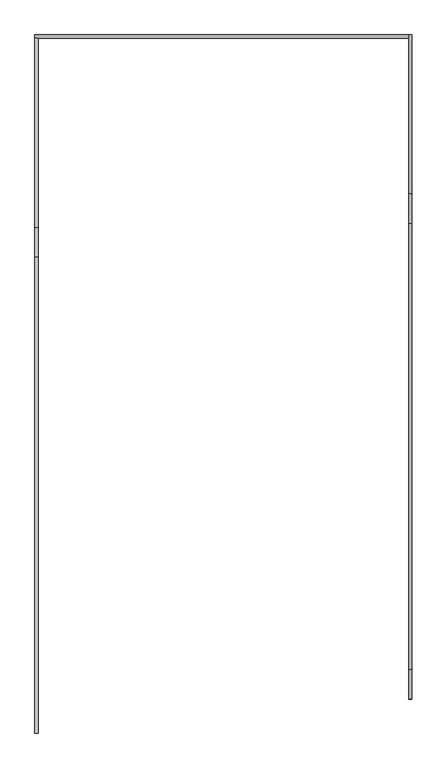
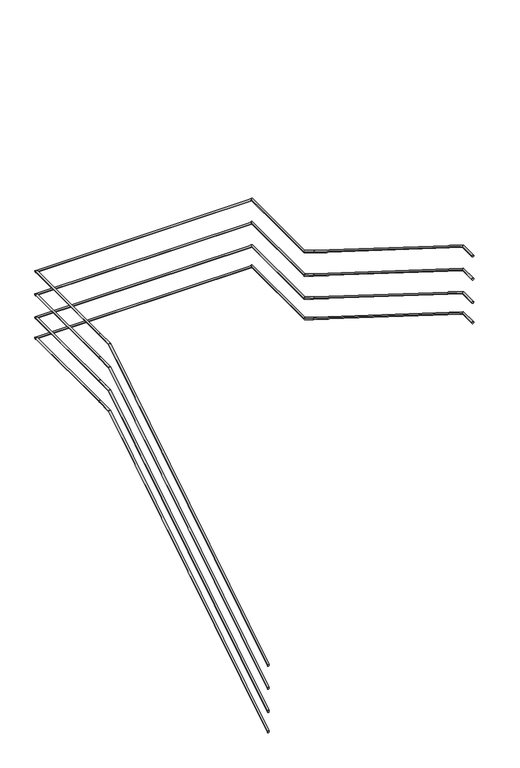
"""IFC4 building model written with IfcOpenShell, lengths in millimetres: railing geometry."""

from ifc_helpers import new_model, si_unit, frame, origin, place, context, project, spatial, circle_curve, ellipse_curve, source, transform, mapped, element, save
from ifc_brep_helpers import plane_surface, cylinder_surface, advanced_brep


def railing_8161422b(model_context):
    return source(origin(), model_context, "Body", "AdvancedBrep", [
        advanced_brep(
        [(51115.4, 10964.5208589, 1508.0091814), (51085.4, 10964.5208589, 1508.0091814), (51115.4, 15448.8385799, 4322.8406512), (51085.4, 15448.8385799, 4322.8406512), (51115.4, 15724.5208589, 4322.8406512), (51085.4, 15724.5208589, 4322.8406512)],
        [
            (0, 1, ellipse_curve(frame((51100.4, 10964.5208589, 1508.0091814), z_axis=(0.0, -1.0, 0.0), x_axis=(0.0, 0.0, -1.0)), 17.7102578, 15.0)),
            (1, 0, ellipse_curve(frame((51100.4, 10964.5208589, 1508.0091814), z_axis=(0.0, -1.0, 0.0), x_axis=(0.0, 0.0, -1.0)), 17.7102578, 15.0)),
            (0, 2),
            (2, 3, ellipse_curve(frame((51100.4, 15448.8385799, 4322.8406512), z_axis=(0.0, -0.9609804318330746, -0.27661635821823227), x_axis=(0.0, 0.27661635821823216, -0.9609804318330747)), 15.6090587, 15.0)),
            (3, 1),
            (3, 2, ellipse_curve(frame((51100.4, 15448.8385799, 4322.8406512), z_axis=(0.0, -0.9609804318330746, -0.27661635821823227), x_axis=(0.0, 0.27661635821823216, -0.9609804318330747)), 15.6090587, 15.0)),
            (4, 5, circle_curve(frame((51100.4, 15724.5208589, 4322.8406512), z_axis=(0.0, 1.0, 0.0), x_axis=(-1.0, 0.0, 0.0)), 15.0)),
            (5, 4, circle_curve(frame((51100.4, 15724.5208589, 4322.8406512), z_axis=(0.0, 1.0, 0.0), x_axis=(-1.0, 0.0, 0.0)), 15.0)),
            (2, 4),
            (5, 3),
        ],
        [
            plane_surface(frame((51100.4, 10964.5208589, 1525.7194391), z_axis=(0.0, -1.0, 0.0), x_axis=(0.0, 0.0, 1.0))),
            cylinder_surface(frame((51100.4, 10972.4955461, 1513.0149374), z_axis=(0.0, -0.8469667807321652, -0.5316458147452987), x_axis=(-1.0, 0.0, 0.0)), 15.0),
            plane_surface(frame((51100.4, 15724.5208589, 4337.8406512), z_axis=(0.0, 1.0, 0.0), x_axis=(0.0, 0.0, 1.0))),
            cylinder_surface(frame((51100.4, 15444.5208589, 4322.8406512), z_axis=(0.0, -1.0, 0.0), x_axis=(-1.0, 0.0, 0.0)), 15.0),
        ],
        [
            (0, [[1, 2]]),
            (1, [[-1, 3, 4, 5]]),
            (1, [[-2, -5, 6, -3]]),
            (2, [[7, 8]]),
            (3, [[-4, 9, -8, 10]]),
            (3, [[-6, -10, -7, -9]]),
        ],
    ),
        advanced_brep(
        [(51115.4, 15724.5208589, 4322.8406512), (51085.4, 15724.5208589, 4322.8406512), (51115.4, 17509.1208589, 4322.8406512), (51085.4, 17509.1208589, 4322.8406512)],
        [
            (0, 1, circle_curve(frame((51100.4, 15724.5208589, 4322.8406512), z_axis=(0.0, -1.0, 0.0), x_axis=(-1.0, 0.0, 0.0)), 15.0)),
            (1, 0, circle_curve(frame((51100.4, 15724.5208589, 4322.8406512), z_axis=(0.0, -1.0, 0.0), x_axis=(-1.0, 0.0, 0.0)), 15.0)),
            (2, 3, circle_curve(frame((51100.4, 17509.1208589, 4322.8406512), z_axis=(0.0, 1.0, 0.0), x_axis=(-1.0, 0.0, 0.0)), 15.0)),
            (3, 2, circle_curve(frame((51100.4, 17509.1208589, 4322.8406512), z_axis=(0.0, 1.0, 0.0), x_axis=(-1.0, 0.0, 0.0)), 15.0)),
            (0, 2),
            (3, 1),
        ],
        [
            plane_surface(frame((51100.4, 15724.5208589, 4337.8406512), z_axis=(0.0, -1.0, 0.0), x_axis=(0.0, 0.0, 1.0))),
            plane_surface(frame((51100.4, 17509.1208589, 4337.8406512), z_axis=(0.0, 1.0, 0.0), x_axis=(0.0, 0.0, 1.0))),
            cylinder_surface(frame((51100.4, 15724.5208589, 4322.8406512), z_axis=(0.0, -1.0, 0.0), x_axis=(-1.0, 0.0, 0.0)), 15.0),
        ],
        [
            (0, [[1, 2]]),
            (1, [[3, 4]]),
            (2, [[-1, 5, -4, 6]]),
            (2, [[-2, -6, -3, -5]]),
        ],
    ),
        advanced_brep(
        [(51085.4, 17509.1208589, 4322.8406512), (51085.4, 17539.1208589, 4322.8406512), (54609.6, 17509.1208589, 4322.8406512), (54609.6, 17539.1208589, 4322.8406512)],
        [
            (0, 1, circle_curve(frame((51085.4, 17524.1208589, 4322.8406512), z_axis=(-1.0, 0.0, 0.0), x_axis=(0.0, 1.0, 0.0)), 15.0)),
            (1, 0, circle_curve(frame((51085.4, 17524.1208589, 4322.8406512), z_axis=(-1.0, 0.0, 0.0), x_axis=(0.0, 1.0, 0.0)), 15.0)),
            (2, 3, circle_curve(frame((54609.6, 17524.1208589, 4322.8406512), z_axis=(1.0, 0.0, 0.0), x_axis=(0.0, 1.0, 0.0)), 15.0)),
            (3, 2, circle_curve(frame((54609.6, 17524.1208589, 4322.8406512), z_axis=(1.0, 0.0, 0.0), x_axis=(0.0, 1.0, 0.0)), 15.0)),
            (0, 2),
            (3, 1),
        ],
        [
            plane_surface(frame((51085.4, 17524.1208589, 4337.8406512), z_axis=(-1.0, 0.0, 0.0), x_axis=(0.0, 1.0, 0.0))),
            plane_surface(frame((54609.6, 17524.1208589, 4337.8406512), z_axis=(1.0, 0.0, 0.0), x_axis=(0.0, 1.0, 0.0))),
            cylinder_surface(frame((51085.4, 17524.1208589, 4322.8406512), z_axis=(-1.0, 0.0, 0.0), x_axis=(0.0, 1.0, 0.0)), 15.0),
        ],
        [
            (0, [[1, 2]]),
            (1, [[3, 4]]),
            (2, [[-1, 5, -4, 6]]),
            (2, [[-2, -6, -3, -5]]),
        ],
    ),
        advanced_brep(
        [(54609.6, 17539.1208589, 4322.8406512), (54639.6, 17539.1208589, 4322.8406512), (54609.6, 16040.2031379, 4322.8406512), (54639.6, 16040.2031379, 4322.8406512), (54609.6, 15764.5208589, 4495.8879692), (54639.6, 15764.5208589, 4495.8879692)],
        [
            (0, 1, circle_curve(frame((54624.6, 17539.1208589, 4322.8406512), z_axis=(0.0, 1.0, 0.0), x_axis=(1.0, 0.0, 0.0)), 15.0)),
            (1, 0, circle_curve(frame((54624.6, 17539.1208589, 4322.8406512), z_axis=(0.0, 1.0, 0.0), x_axis=(1.0, 0.0, 0.0)), 15.0)),
            (0, 2),
            (2, 3, ellipse_curve(frame((54624.6, 16040.2031379, 4322.8406512), z_axis=(0.0, 0.9609804318330746, -0.27661635821823227), x_axis=(0.0, 0.2766163582182326, 0.9609804318330746)), 15.6090587, 15.0)),
            (3, 1),
            (3, 2, ellipse_curve(frame((54624.6, 16040.2031379, 4322.8406512), z_axis=(0.0, 0.9609804318330746, -0.27661635821823227), x_axis=(0.0, 0.2766163582182326, 0.9609804318330746)), 15.6090587, 15.0)),
            (4, 5, ellipse_curve(frame((54624.6, 15764.5208589, 4495.8879692), z_axis=(0.0, -1.0, 0.0), x_axis=(0.0, 0.0, -1.0)), 17.7102578, 15.0)),
            (5, 4, ellipse_curve(frame((54624.6, 15764.5208589, 4495.8879692), z_axis=(0.0, -1.0, 0.0), x_axis=(0.0, 0.0, -1.0)), 17.7102578, 15.0)),
            (2, 4),
            (5, 3),
        ],
        [
            plane_surface(frame((54624.6, 17539.1208589, 4337.8406512), z_axis=(0.0, 1.0, 0.0), x_axis=(0.0, 0.0, -1.0))),
            cylinder_surface(frame((54624.6, 17539.1208589, 4322.8406512), z_axis=(0.0, 1.0, 0.0), x_axis=(1.0, 0.0, 0.0)), 15.0),
            plane_surface(frame((54624.6, 15764.5208589, 4513.598227), z_axis=(0.0, -1.0, 0.0), x_axis=(0.0, 0.0, -1.0))),
            cylinder_surface(frame((54624.6, 16036.5461717, 4325.1361495), z_axis=(0.0, 0.8469667807321651, -0.5316458147452987), x_axis=(1.0, 0.0, 0.0)), 15.0),
        ],
        [
            (0, [[1, 2]]),
            (1, [[-1, 3, 4, 5]]),
            (1, [[-2, -5, 6, -3]]),
            (2, [[7, 8]]),
            (3, [[-4, 9, -8, 10]]),
            (3, [[-6, -10, -7, -9]]),
        ],
    ),
        advanced_brep(
        [(54609.6, 15764.5208589, 4495.8879692), (54639.6, 15764.5208589, 4495.8879692), (54609.6, 11560.2031379, 7134.9618634), (54639.6, 11560.2031379, 7134.9618634), (54609.6, 11284.5208589, 7134.9618634), (54639.6, 11284.5208589, 7134.9618634)],
        [
            (0, 1, ellipse_curve(frame((54624.6, 15764.5208589, 4495.8879692), z_axis=(0.0, 1.0, 0.0), x_axis=(0.0, 0.0, -1.0)), 17.7102578, 15.0)),
            (1, 0, ellipse_curve(frame((54624.6, 15764.5208589, 4495.8879692), z_axis=(0.0, 1.0, 0.0), x_axis=(0.0, 0.0, -1.0)), 17.7102578, 15.0)),
            (0, 2),
            (2, 3, ellipse_curve(frame((54624.6, 11560.2031379, 7134.9618634), z_axis=(0.0, 0.9609804318330746, -0.2766163582182322), x_axis=(0.0, -0.2766163582182318, -0.9609804318330748)), 15.6090587, 15.0)),
            (3, 1),
            (3, 2, ellipse_curve(frame((54624.6, 11560.2031379, 7134.9618634), z_axis=(0.0, 0.9609804318330746, -0.2766163582182322), x_axis=(0.0, -0.2766163582182318, -0.9609804318330748)), 15.6090587, 15.0)),
            (4, 5, circle_curve(frame((54624.6, 11284.5208589, 7134.9618634), z_axis=(0.0, -1.0, 0.0), x_axis=(1.0, 0.0, 0.0)), 15.0)),
            (5, 4, circle_curve(frame((54624.6, 11284.5208589, 7134.9618634), z_axis=(0.0, -1.0, 0.0), x_axis=(1.0, 0.0, 0.0)), 15.0)),
            (2, 4),
            (5, 3),
        ],
        [
            plane_surface(frame((54624.6, 15764.5208589, 4513.598227), z_axis=(0.0, 1.0, 0.0), x_axis=(0.0, 0.0, -1.0))),
            cylinder_surface(frame((54624.6, 15756.5461717, 4500.8937253), z_axis=(0.0, 0.8469667807321652, -0.5316458147452986), x_axis=(1.0, 0.0, 0.0)), 15.0),
            plane_surface(frame((54624.6, 11284.5208589, 7149.9618634), z_axis=(0.0, -1.0, 0.0), x_axis=(0.0, 0.0, -1.0))),
            cylinder_surface(frame((54624.6, 11564.5208589, 7134.9618634), z_axis=(0.0, 1.0, 0.0), x_axis=(1.0, 0.0, 0.0)), 15.0),
        ],
        [
            (0, [[1, 2]]),
            (1, [[-1, 3, 4, 5]]),
            (1, [[-2, -5, 6, -3]]),
            (2, [[7, 8]]),
            (3, [[-4, 9, -8, 10]]),
            (3, [[-6, -10, -7, -9]]),
        ],
    ),
        advanced_brep(
        [(51115.4, 10964.5208589, 708.0091814), (51085.4, 10964.5208589, 708.0091814), (51115.4, 15448.8385799, 3522.8406512), (51085.4, 15448.8385799, 3522.8406512), (51115.4, 15724.5208589, 3522.8406512), (51085.4, 15724.5208589, 3522.8406512)],
        [
            (0, 1, ellipse_curve(frame((51100.4, 10964.5208589, 708.0091814), z_axis=(0.0, -1.0, 0.0), x_axis=(0.0, 0.0, -1.0)), 17.7102578, 15.0)),
            (1, 0, ellipse_curve(frame((51100.4, 10964.5208589, 708.0091814), z_axis=(0.0, -1.0, 0.0), x_axis=(0.0, 0.0, -1.0)), 17.7102578, 15.0)),
            (0, 2),
            (2, 3, ellipse_curve(frame((51100.4, 15448.8385799, 3522.8406512), z_axis=(0.0, -0.9609804318330746, -0.27661635821823227), x_axis=(0.0, 0.27661635821823216, -0.9609804318330747)), 15.6090587, 15.0)),
            (3, 1),
            (3, 2, ellipse_curve(frame((51100.4, 15448.8385799, 3522.8406512), z_axis=(0.0, -0.9609804318330746, -0.27661635821823227), x_axis=(0.0, 0.27661635821823216, -0.9609804318330747)), 15.6090587, 15.0)),
            (4, 5, circle_curve(frame((51100.4, 15724.5208589, 3522.8406512), z_axis=(0.0, 1.0, 0.0), x_axis=(-1.0, 0.0, 0.0)), 15.0)),
            (5, 4, circle_curve(frame((51100.4, 15724.5208589, 3522.8406512), z_axis=(0.0, 1.0, 0.0), x_axis=(-1.0, 0.0, 0.0)), 15.0)),
            (2, 4),
            (5, 3),
        ],
        [
            plane_surface(frame((51100.4, 10964.5208589, 725.7194391), z_axis=(0.0, -1.0, 0.0), x_axis=(0.0, 0.0, 1.0))),
            cylinder_surface(frame((51100.4, 10972.4955461, 713.0149374), z_axis=(0.0, -0.8469667807321652, -0.5316458147452987), x_axis=(-1.0, 0.0, 0.0)), 15.0),
            plane_surface(frame((51100.4, 15724.5208589, 3537.8406512), z_axis=(0.0, 1.0, 0.0), x_axis=(0.0, 0.0, 1.0))),
            cylinder_surface(frame((51100.4, 15444.5208589, 3522.8406512), z_axis=(0.0, -1.0, 0.0), x_axis=(-1.0, 0.0, 0.0)), 15.0),
        ],
        [
            (0, [[1, 2]]),
            (1, [[-1, 3, 4, 5]]),
            (1, [[-2, -5, 6, -3]]),
            (2, [[7, 8]]),
            (3, [[-4, 9, -8, 10]]),
            (3, [[-6, -10, -7, -9]]),
        ],
    ),
        advanced_brep(
        [(51115.4, 15724.5208589, 3522.8406512), (51085.4, 15724.5208589, 3522.8406512), (51115.4, 17509.1208589, 3522.8406512), (51085.4, 17509.1208589, 3522.8406512)],
        [
            (0, 1, circle_curve(frame((51100.4, 15724.5208589, 3522.8406512), z_axis=(0.0, -1.0, 0.0), x_axis=(-1.0, 0.0, 0.0)), 15.0)),
            (1, 0, circle_curve(frame((51100.4, 15724.5208589, 3522.8406512), z_axis=(0.0, -1.0, 0.0), x_axis=(-1.0, 0.0, 0.0)), 15.0)),
            (2, 3, circle_curve(frame((51100.4, 17509.1208589, 3522.8406512), z_axis=(0.0, 1.0, 0.0), x_axis=(-1.0, 0.0, 0.0)), 15.0)),
            (3, 2, circle_curve(frame((51100.4, 17509.1208589, 3522.8406512), z_axis=(0.0, 1.0, 0.0), x_axis=(-1.0, 0.0, 0.0)), 15.0)),
            (0, 2),
            (3, 1),
        ],
        [
            plane_surface(frame((51100.4, 15724.5208589, 3537.8406512), z_axis=(0.0, -1.0, 0.0), x_axis=(0.0, 0.0, 1.0))),
            plane_surface(frame((51100.4, 17509.1208589, 3537.8406512), z_axis=(0.0, 1.0, 0.0), x_axis=(0.0, 0.0, 1.0))),
            cylinder_surface(frame((51100.4, 15724.5208589, 3522.8406512), z_axis=(0.0, -1.0, 0.0), x_axis=(-1.0, 0.0, 0.0)), 15.0),
        ],
        [
            (0, [[1, 2]]),
            (1, [[3, 4]]),
            (2, [[-1, 5, -4, 6]]),
            (2, [[-2, -6, -3, -5]]),
        ],
    ),
        advanced_brep(
        [(51085.4, 17509.1208589, 3522.8406512), (51085.4, 17539.1208589, 3522.8406512), (54609.6, 17509.1208589, 3522.8406512), (54609.6, 17539.1208589, 3522.8406512)],
        [
            (0, 1, circle_curve(frame((51085.4, 17524.1208589, 3522.8406512), z_axis=(-1.0, 0.0, 0.0), x_axis=(0.0, 1.0, 0.0)), 15.0)),
            (1, 0, circle_curve(frame((51085.4, 17524.1208589, 3522.8406512), z_axis=(-1.0, 0.0, 0.0), x_axis=(0.0, 1.0, 0.0)), 15.0)),
            (2, 3, circle_curve(frame((54609.6, 17524.1208589, 3522.8406512), z_axis=(1.0, 0.0, 0.0), x_axis=(0.0, 1.0, 0.0)), 15.0)),
            (3, 2, circle_curve(frame((54609.6, 17524.1208589, 3522.8406512), z_axis=(1.0, 0.0, 0.0), x_axis=(0.0, 1.0, 0.0)), 15.0)),
            (0, 2),
            (3, 1),
        ],
        [
            plane_surface(frame((51085.4, 17524.1208589, 3537.8406512), z_axis=(-1.0, 0.0, 0.0), x_axis=(0.0, 1.0, 0.0))),
            plane_surface(frame((54609.6, 17524.1208589, 3537.8406512), z_axis=(1.0, 0.0, 0.0), x_axis=(0.0, 1.0, 0.0))),
            cylinder_surface(frame((51085.4, 17524.1208589, 3522.8406512), z_axis=(-1.0, 0.0, 0.0), x_axis=(0.0, 1.0, 0.0)), 15.0),
        ],
        [
            (0, [[1, 2]]),
            (1, [[3, 4]]),
            (2, [[-1, 5, -4, 6]]),
            (2, [[-2, -6, -3, -5]]),
        ],
    ),
        advanced_brep(
        [(54609.6, 17539.1208589, 3522.8406512), (54639.6, 17539.1208589, 3522.8406512), (54609.6, 16040.2031379, 3522.8406512), (54639.6, 16040.2031379, 3522.8406512), (54609.6, 15764.5208589, 3695.8879692), (54639.6, 15764.5208589, 3695.8879692)],
        [
            (0, 1, circle_curve(frame((54624.6, 17539.1208589, 3522.8406512), z_axis=(0.0, 1.0, 0.0), x_axis=(1.0, 0.0, 0.0)), 15.0)),
            (1, 0, circle_curve(frame((54624.6, 17539.1208589, 3522.8406512), z_axis=(0.0, 1.0, 0.0), x_axis=(1.0, 0.0, 0.0)), 15.0)),
            (0, 2),
            (2, 3, ellipse_curve(frame((54624.6, 16040.2031379, 3522.8406512), z_axis=(0.0, 0.9609804318330746, -0.27661635821823227), x_axis=(0.0, 0.2766163582182326, 0.9609804318330746)), 15.6090587, 15.0)),
            (3, 1),
            (3, 2, ellipse_curve(frame((54624.6, 16040.2031379, 3522.8406512), z_axis=(0.0, 0.9609804318330746, -0.27661635821823227), x_axis=(0.0, 0.2766163582182326, 0.9609804318330746)), 15.6090587, 15.0)),
            (4, 5, ellipse_curve(frame((54624.6, 15764.5208589, 3695.8879692), z_axis=(0.0, -1.0, 0.0), x_axis=(0.0, 0.0, -1.0)), 17.7102578, 15.0)),
            (5, 4, ellipse_curve(frame((54624.6, 15764.5208589, 3695.8879692), z_axis=(0.0, -1.0, 0.0), x_axis=(0.0, 0.0, -1.0)), 17.7102578, 15.0)),
            (2, 4),
            (5, 3),
        ],
        [
            plane_surface(frame((54624.6, 17539.1208589, 3537.8406512), z_axis=(0.0, 1.0, 0.0), x_axis=(0.0, 0.0, -1.0))),
            cylinder_surface(frame((54624.6, 17539.1208589, 3522.8406512), z_axis=(0.0, 1.0, 0.0), x_axis=(1.0, 0.0, 0.0)), 15.0),
            plane_surface(frame((54624.6, 15764.5208589, 3713.598227), z_axis=(0.0, -1.0, 0.0), x_axis=(0.0, 0.0, -1.0))),
            cylinder_surface(frame((54624.6, 16036.5461717, 3525.1361495), z_axis=(0.0, 0.8469667807321651, -0.5316458147452987), x_axis=(1.0, 0.0, 0.0)), 15.0),
        ],
        [
            (0, [[1, 2]]),
            (1, [[-1, 3, 4, 5]]),
            (1, [[-2, -5, 6, -3]]),
            (2, [[7, 8]]),
            (3, [[-4, 9, -8, 10]]),
            (3, [[-6, -10, -7, -9]]),
        ],
    ),
        advanced_brep(
        [(54609.6, 15764.5208589, 3695.8879692), (54639.6, 15764.5208589, 3695.8879692), (54609.6, 11560.2031379, 6334.9618634), (54639.6, 11560.2031379, 6334.9618634), (54609.6, 11284.5208589, 6334.9618634), (54639.6, 11284.5208589, 6334.9618634)],
        [
            (0, 1, ellipse_curve(frame((54624.6, 15764.5208589, 3695.8879692), z_axis=(0.0, 1.0, 0.0), x_axis=(0.0, 0.0, -1.0)), 17.7102578, 15.0)),
            (1, 0, ellipse_curve(frame((54624.6, 15764.5208589, 3695.8879692), z_axis=(0.0, 1.0, 0.0), x_axis=(0.0, 0.0, -1.0)), 17.7102578, 15.0)),
            (0, 2),
            (2, 3, ellipse_curve(frame((54624.6, 11560.2031379, 6334.9618634), z_axis=(0.0, 0.9609804318330746, -0.2766163582182322), x_axis=(0.0, -0.2766163582182318, -0.9609804318330748)), 15.6090587, 15.0)),
            (3, 1),
            (3, 2, ellipse_curve(frame((54624.6, 11560.2031379, 6334.9618634), z_axis=(0.0, 0.9609804318330746, -0.2766163582182322), x_axis=(0.0, -0.2766163582182318, -0.9609804318330748)), 15.6090587, 15.0)),
            (4, 5, circle_curve(frame((54624.6, 11284.5208589, 6334.9618634), z_axis=(0.0, -1.0, 0.0), x_axis=(1.0, 0.0, 0.0)), 15.0)),
            (5, 4, circle_curve(frame((54624.6, 11284.5208589, 6334.9618634), z_axis=(0.0, -1.0, 0.0), x_axis=(1.0, 0.0, 0.0)), 15.0)),
            (2, 4),
            (5, 3),
        ],
        [
            plane_surface(frame((54624.6, 15764.5208589, 3713.598227), z_axis=(0.0, 1.0, 0.0), x_axis=(0.0, 0.0, -1.0))),
            cylinder_surface(frame((54624.6, 15756.5461717, 3700.8937253), z_axis=(0.0, 0.8469667807321652, -0.5316458147452986), x_axis=(1.0, 0.0, 0.0)), 15.0),
            plane_surface(frame((54624.6, 11284.5208589, 6349.9618634), z_axis=(0.0, -1.0, 0.0), x_axis=(0.0, 0.0, -1.0))),
            cylinder_surface(frame((54624.6, 11564.5208589, 6334.9618634), z_axis=(0.0, 1.0, 0.0), x_axis=(1.0, 0.0, 0.0)), 15.0),
        ],
        [
            (0, [[1, 2]]),
            (1, [[-1, 3, 4, 5]]),
            (1, [[-2, -5, 6, -3]]),
            (2, [[7, 8]]),
            (3, [[-4, 9, -8, 10]]),
            (3, [[-6, -10, -7, -9]]),
        ],
    ),
        advanced_brep(
        [(51115.4, 10964.5208589, 1108.0091814), (51085.4, 10964.5208589, 1108.0091814), (51115.4, 15448.8385799, 3922.8406512), (51085.4, 15448.8385799, 3922.8406512), (51115.4, 15724.5208589, 3922.8406512), (51085.4, 15724.5208589, 3922.8406512)],
        [
            (0, 1, ellipse_curve(frame((51100.4, 10964.5208589, 1108.0091814), z_axis=(0.0, -1.0, 0.0), x_axis=(0.0, 0.0, -1.0)), 17.7102578, 15.0)),
            (1, 0, ellipse_curve(frame((51100.4, 10964.5208589, 1108.0091814), z_axis=(0.0, -1.0, 0.0), x_axis=(0.0, 0.0, -1.0)), 17.7102578, 15.0)),
            (0, 2),
            (2, 3, ellipse_curve(frame((51100.4, 15448.8385799, 3922.8406512), z_axis=(0.0, -0.9609804318330746, -0.27661635821823227), x_axis=(0.0, 0.27661635821823216, -0.9609804318330747)), 15.6090587, 15.0)),
            (3, 1),
            (3, 2, ellipse_curve(frame((51100.4, 15448.8385799, 3922.8406512), z_axis=(0.0, -0.9609804318330746, -0.27661635821823227), x_axis=(0.0, 0.27661635821823216, -0.9609804318330747)), 15.6090587, 15.0)),
            (4, 5, circle_curve(frame((51100.4, 15724.5208589, 3922.8406512), z_axis=(0.0, 1.0, 0.0), x_axis=(-1.0, 0.0, 0.0)), 15.0)),
            (5, 4, circle_curve(frame((51100.4, 15724.5208589, 3922.8406512), z_axis=(0.0, 1.0, 0.0), x_axis=(-1.0, 0.0, 0.0)), 15.0)),
            (2, 4),
            (5, 3),
        ],
        [
            plane_surface(frame((51100.4, 10964.5208589, 1125.7194391), z_axis=(0.0, -1.0, 0.0), x_axis=(0.0, 0.0, 1.0))),
            cylinder_surface(frame((51100.4, 10972.4955461, 1113.0149374), z_axis=(0.0, -0.8469667807321652, -0.5316458147452987), x_axis=(-1.0, 0.0, 0.0)), 15.0),
            plane_surface(frame((51100.4, 15724.5208589, 3937.8406512), z_axis=(0.0, 1.0, 0.0), x_axis=(0.0, 0.0, 1.0))),
            cylinder_surface(frame((51100.4, 15444.5208589, 3922.8406512), z_axis=(0.0, -1.0, 0.0), x_axis=(-1.0, 0.0, 0.0)), 15.0),
        ],
        [
            (0, [[1, 2]]),
            (1, [[-1, 3, 4, 5]]),
            (1, [[-2, -5, 6, -3]]),
            (2, [[7, 8]]),
            (3, [[-4, 9, -8, 10]]),
            (3, [[-6, -10, -7, -9]]),
        ],
    ),
        advanced_brep(
        [(51115.4, 15724.5208589, 3922.8406512), (51085.4, 15724.5208589, 3922.8406512), (51115.4, 17509.1208589, 3922.8406512), (51085.4, 17509.1208589, 3922.8406512)],
        [
            (0, 1, circle_curve(frame((51100.4, 15724.5208589, 3922.8406512), z_axis=(0.0, -1.0, 0.0), x_axis=(-1.0, 0.0, 0.0)), 15.0)),
            (1, 0, circle_curve(frame((51100.4, 15724.5208589, 3922.8406512), z_axis=(0.0, -1.0, 0.0), x_axis=(-1.0, 0.0, 0.0)), 15.0)),
            (2, 3, circle_curve(frame((51100.4, 17509.1208589, 3922.8406512), z_axis=(0.0, 1.0, 0.0), x_axis=(-1.0, 0.0, 0.0)), 15.0)),
            (3, 2, circle_curve(frame((51100.4, 17509.1208589, 3922.8406512), z_axis=(0.0, 1.0, 0.0), x_axis=(-1.0, 0.0, 0.0)), 15.0)),
            (0, 2),
            (3, 1),
        ],
        [
            plane_surface(frame((51100.4, 15724.5208589, 3937.8406512), z_axis=(0.0, -1.0, 0.0), x_axis=(0.0, 0.0, 1.0))),
            plane_surface(frame((51100.4, 17509.1208589, 3937.8406512), z_axis=(0.0, 1.0, 0.0), x_axis=(0.0, 0.0, 1.0))),
            cylinder_surface(frame((51100.4, 15724.5208589, 3922.8406512), z_axis=(0.0, -1.0, 0.0), x_axis=(-1.0, 0.0, 0.0)), 15.0),
        ],
        [
            (0, [[1, 2]]),
            (1, [[3, 4]]),
            (2, [[-1, 5, -4, 6]]),
            (2, [[-2, -6, -3, -5]]),
        ],
    ),
        advanced_brep(
        [(51085.4, 17509.1208589, 3922.8406512), (51085.4, 17539.1208589, 3922.8406512), (54609.6, 17509.1208589, 3922.8406512), (54609.6, 17539.1208589, 3922.8406512)],
        [
            (0, 1, circle_curve(frame((51085.4, 17524.1208589, 3922.8406512), z_axis=(-1.0, 0.0, 0.0), x_axis=(0.0, 1.0, 0.0)), 15.0)),
            (1, 0, circle_curve(frame((51085.4, 17524.1208589, 3922.8406512), z_axis=(-1.0, 0.0, 0.0), x_axis=(0.0, 1.0, 0.0)), 15.0)),
            (2, 3, circle_curve(frame((54609.6, 17524.1208589, 3922.8406512), z_axis=(1.0, 0.0, 0.0), x_axis=(0.0, 1.0, 0.0)), 15.0)),
            (3, 2, circle_curve(frame((54609.6, 17524.1208589, 3922.8406512), z_axis=(1.0, 0.0, 0.0), x_axis=(0.0, 1.0, 0.0)), 15.0)),
            (0, 2),
            (3, 1),
        ],
        [
            plane_surface(frame((51085.4, 17524.1208589, 3937.8406512), z_axis=(-1.0, 0.0, 0.0), x_axis=(0.0, 1.0, 0.0))),
            plane_surface(frame((54609.6, 17524.1208589, 3937.8406512), z_axis=(1.0, 0.0, 0.0), x_axis=(0.0, 1.0, 0.0))),
            cylinder_surface(frame((51085.4, 17524.1208589, 3922.8406512), z_axis=(-1.0, 0.0, 0.0), x_axis=(0.0, 1.0, 0.0)), 15.0),
        ],
        [
            (0, [[1, 2]]),
            (1, [[3, 4]]),
            (2, [[-1, 5, -4, 6]]),
            (2, [[-2, -6, -3, -5]]),
        ],
    ),
        advanced_brep(
        [(54609.6, 17539.1208589, 3922.8406512), (54639.6, 17539.1208589, 3922.8406512), (54609.6, 16040.2031379, 3922.8406512), (54639.6, 16040.2031379, 3922.8406512), (54609.6, 15764.5208589, 4095.8879692), (54639.6, 15764.5208589, 4095.8879692)],
        [
            (0, 1, circle_curve(frame((54624.6, 17539.1208589, 3922.8406512), z_axis=(0.0, 1.0, 0.0), x_axis=(1.0, 0.0, 0.0)), 15.0)),
            (1, 0, circle_curve(frame((54624.6, 17539.1208589, 3922.8406512), z_axis=(0.0, 1.0, 0.0), x_axis=(1.0, 0.0, 0.0)), 15.0)),
            (0, 2),
            (2, 3, ellipse_curve(frame((54624.6, 16040.2031379, 3922.8406512), z_axis=(0.0, 0.9609804318330746, -0.27661635821823227), x_axis=(0.0, 0.2766163582182326, 0.9609804318330746)), 15.6090587, 15.0)),
            (3, 1),
            (3, 2, ellipse_curve(frame((54624.6, 16040.2031379, 3922.8406512), z_axis=(0.0, 0.9609804318330746, -0.27661635821823227), x_axis=(0.0, 0.2766163582182326, 0.9609804318330746)), 15.6090587, 15.0)),
            (4, 5, ellipse_curve(frame((54624.6, 15764.5208589, 4095.8879692), z_axis=(0.0, -1.0, 0.0), x_axis=(0.0, 0.0, -1.0)), 17.7102578, 15.0)),
            (5, 4, ellipse_curve(frame((54624.6, 15764.5208589, 4095.8879692), z_axis=(0.0, -1.0, 0.0), x_axis=(0.0, 0.0, -1.0)), 17.7102578, 15.0)),
            (2, 4),
            (5, 3),
        ],
        [
            plane_surface(frame((54624.6, 17539.1208589, 3937.8406512), z_axis=(0.0, 1.0, 0.0), x_axis=(0.0, 0.0, -1.0))),
            cylinder_surface(frame((54624.6, 17539.1208589, 3922.8406512), z_axis=(0.0, 1.0, 0.0), x_axis=(1.0, 0.0, 0.0)), 15.0),
            plane_surface(frame((54624.6, 15764.5208589, 4113.598227), z_axis=(0.0, -1.0, 0.0), x_axis=(0.0, 0.0, -1.0))),
            cylinder_surface(frame((54624.6, 16036.5461717, 3925.1361495), z_axis=(0.0, 0.8469667807321651, -0.5316458147452987), x_axis=(1.0, 0.0, 0.0)), 15.0),
        ],
        [
            (0, [[1, 2]]),
            (1, [[-1, 3, 4, 5]]),
            (1, [[-2, -5, 6, -3]]),
            (2, [[7, 8]]),
            (3, [[-4, 9, -8, 10]]),
            (3, [[-6, -10, -7, -9]]),
        ],
    ),
        advanced_brep(
        [(54609.6, 15764.5208589, 4095.8879692), (54639.6, 15764.5208589, 4095.8879692), (54609.6, 11560.2031379, 6734.9618634), (54639.6, 11560.2031379, 6734.9618634), (54609.6, 11284.5208589, 6734.9618634), (54639.6, 11284.5208589, 6734.9618634)],
        [
            (0, 1, ellipse_curve(frame((54624.6, 15764.5208589, 4095.8879692), z_axis=(0.0, 1.0, 0.0), x_axis=(0.0, 0.0, -1.0)), 17.7102578, 15.0)),
            (1, 0, ellipse_curve(frame((54624.6, 15764.5208589, 4095.8879692), z_axis=(0.0, 1.0, 0.0), x_axis=(0.0, 0.0, -1.0)), 17.7102578, 15.0)),
            (0, 2),
            (2, 3, ellipse_curve(frame((54624.6, 11560.2031379, 6734.9618634), z_axis=(0.0, 0.9609804318330746, -0.2766163582182322), x_axis=(0.0, -0.2766163582182318, -0.9609804318330748)), 15.6090587, 15.0)),
            (3, 1),
            (3, 2, ellipse_curve(frame((54624.6, 11560.2031379, 6734.9618634), z_axis=(0.0, 0.9609804318330746, -0.2766163582182322), x_axis=(0.0, -0.2766163582182318, -0.9609804318330748)), 15.6090587, 15.0)),
            (4, 5, circle_curve(frame((54624.6, 11284.5208589, 6734.9618634), z_axis=(0.0, -1.0, 0.0), x_axis=(1.0, 0.0, 0.0)), 15.0)),
            (5, 4, circle_curve(frame((54624.6, 11284.5208589, 6734.9618634), z_axis=(0.0, -1.0, 0.0), x_axis=(1.0, 0.0, 0.0)), 15.0)),
            (2, 4),
            (5, 3),
        ],
        [
            plane_surface(frame((54624.6, 15764.5208589, 4113.598227), z_axis=(0.0, 1.0, 0.0), x_axis=(0.0, 0.0, -1.0))),
            cylinder_surface(frame((54624.6, 15756.5461717, 4100.8937253), z_axis=(0.0, 0.8469667807321652, -0.5316458147452986), x_axis=(1.0, 0.0, 0.0)), 15.0),
            plane_surface(frame((54624.6, 11284.5208589, 6749.9618634), z_axis=(0.0, -1.0, 0.0), x_axis=(0.0, 0.0, -1.0))),
            cylinder_surface(frame((54624.6, 11564.5208589, 6734.9618634), z_axis=(0.0, 1.0, 0.0), x_axis=(1.0, 0.0, 0.0)), 15.0),
        ],
        [
            (0, [[1, 2]]),
            (1, [[-1, 3, 4, 5]]),
            (1, [[-2, -5, 6, -3]]),
            (2, [[7, 8]]),
            (3, [[-4, 9, -8, 10]]),
            (3, [[-6, -10, -7, -9]]),
        ],
    ),
        advanced_brep(
        [(51115.4, 10964.5208589, 358.0091814), (51085.4, 10964.5208589, 358.0091814), (51115.4, 15448.8385799, 3172.8406512), (51085.4, 15448.8385799, 3172.8406512), (51115.4, 15724.5208589, 3172.8406512), (51085.4, 15724.5208589, 3172.8406512)],
        [
            (0, 1, ellipse_curve(frame((51100.4, 10964.5208589, 358.0091814), z_axis=(0.0, -1.0, 0.0), x_axis=(0.0, 0.0, -1.0)), 17.7102578, 15.0)),
            (1, 0, ellipse_curve(frame((51100.4, 10964.5208589, 358.0091814), z_axis=(0.0, -1.0, 0.0), x_axis=(0.0, 0.0, -1.0)), 17.7102578, 15.0)),
            (0, 2),
            (2, 3, ellipse_curve(frame((51100.4, 15448.8385799, 3172.8406512), z_axis=(0.0, -0.9609804318330746, -0.27661635821823227), x_axis=(0.0, 0.27661635821823216, -0.9609804318330747)), 15.6090587, 15.0)),
            (3, 1),
            (3, 2, ellipse_curve(frame((51100.4, 15448.8385799, 3172.8406512), z_axis=(0.0, -0.9609804318330746, -0.27661635821823227), x_axis=(0.0, 0.27661635821823216, -0.9609804318330747)), 15.6090587, 15.0)),
            (4, 5, circle_curve(frame((51100.4, 15724.5208589, 3172.8406512), z_axis=(0.0, 1.0, 0.0), x_axis=(-1.0, 0.0, 0.0)), 15.0)),
            (5, 4, circle_curve(frame((51100.4, 15724.5208589, 3172.8406512), z_axis=(0.0, 1.0, 0.0), x_axis=(-1.0, 0.0, 0.0)), 15.0)),
            (2, 4),
            (5, 3),
        ],
        [
            plane_surface(frame((51100.4, 10964.5208589, 375.7194391), z_axis=(0.0, -1.0, 0.0), x_axis=(0.0, 0.0, 1.0))),
            cylinder_surface(frame((51100.4, 10972.4955461, 363.0149374), z_axis=(0.0, -0.8469667807321652, -0.5316458147452987), x_axis=(-1.0, 0.0, 0.0)), 15.0),
            plane_surface(frame((51100.4, 15724.5208589, 3187.8406512), z_axis=(0.0, 1.0, 0.0), x_axis=(0.0, 0.0, 1.0))),
            cylinder_surface(frame((51100.4, 15444.5208589, 3172.8406512), z_axis=(0.0, -1.0, 0.0), x_axis=(-1.0, 0.0, 0.0)), 15.0),
        ],
        [
            (0, [[1, 2]]),
            (1, [[-1, 3, 4, 5]]),
            (1, [[-2, -5, 6, -3]]),
            (2, [[7, 8]]),
            (3, [[-4, 9, -8, 10]]),
            (3, [[-6, -10, -7, -9]]),
        ],
    ),
        advanced_brep(
        [(51115.4, 15724.5208589, 3172.8406512), (51085.4, 15724.5208589, 3172.8406512), (51115.4, 17509.1208589, 3172.8406512), (51085.4, 17509.1208589, 3172.8406512)],
        [
            (0, 1, circle_curve(frame((51100.4, 15724.5208589, 3172.8406512), z_axis=(0.0, -1.0, 0.0), x_axis=(-1.0, 0.0, 0.0)), 15.0)),
            (1, 0, circle_curve(frame((51100.4, 15724.5208589, 3172.8406512), z_axis=(0.0, -1.0, 0.0), x_axis=(-1.0, 0.0, 0.0)), 15.0)),
            (2, 3, circle_curve(frame((51100.4, 17509.1208589, 3172.8406512), z_axis=(0.0, 1.0, 0.0), x_axis=(-1.0, 0.0, 0.0)), 15.0)),
            (3, 2, circle_curve(frame((51100.4, 17509.1208589, 3172.8406512), z_axis=(0.0, 1.0, 0.0), x_axis=(-1.0, 0.0, 0.0)), 15.0)),
            (0, 2),
            (3, 1),
        ],
        [
            plane_surface(frame((51100.4, 15724.5208589, 3187.8406512), z_axis=(0.0, -1.0, 0.0), x_axis=(0.0, 0.0, 1.0))),
            plane_surface(frame((51100.4, 17509.1208589, 3187.8406512), z_axis=(0.0, 1.0, 0.0), x_axis=(0.0, 0.0, 1.0))),
            cylinder_surface(frame((51100.4, 15724.5208589, 3172.8406512), z_axis=(0.0, -1.0, 0.0), x_axis=(-1.0, 0.0, 0.0)), 15.0),
        ],
        [
            (0, [[1, 2]]),
            (1, [[3, 4]]),
            (2, [[-1, 5, -4, 6]]),
            (2, [[-2, -6, -3, -5]]),
        ],
    ),
        advanced_brep(
        [(51085.4, 17509.1208589, 3172.8406512), (51085.4, 17539.1208589, 3172.8406512), (54609.6, 17509.1208589, 3172.8406512), (54609.6, 17539.1208589, 3172.8406512)],
        [
            (0, 1, circle_curve(frame((51085.4, 17524.1208589, 3172.8406512), z_axis=(-1.0, 0.0, 0.0), x_axis=(0.0, 1.0, 0.0)), 15.0)),
            (1, 0, circle_curve(frame((51085.4, 17524.1208589, 3172.8406512), z_axis=(-1.0, 0.0, 0.0), x_axis=(0.0, 1.0, 0.0)), 15.0)),
            (2, 3, circle_curve(frame((54609.6, 17524.1208589, 3172.8406512), z_axis=(1.0, 0.0, 0.0), x_axis=(0.0, 1.0, 0.0)), 15.0)),
            (3, 2, circle_curve(frame((54609.6, 17524.1208589, 3172.8406512), z_axis=(1.0, 0.0, 0.0), x_axis=(0.0, 1.0, 0.0)), 15.0)),
            (0, 2),
            (3, 1),
        ],
        [
            plane_surface(frame((51085.4, 17524.1208589, 3187.8406512), z_axis=(-1.0, 0.0, 0.0), x_axis=(0.0, 1.0, 0.0))),
            plane_surface(frame((54609.6, 17524.1208589, 3187.8406512), z_axis=(1.0, 0.0, 0.0), x_axis=(0.0, 1.0, 0.0))),
            cylinder_surface(frame((51085.4, 17524.1208589, 3172.8406512), z_axis=(-1.0, 0.0, 0.0), x_axis=(0.0, 1.0, 0.0)), 15.0),
        ],
        [
            (0, [[1, 2]]),
            (1, [[3, 4]]),
            (2, [[-1, 5, -4, 6]]),
            (2, [[-2, -6, -3, -5]]),
        ],
    ),
        advanced_brep(
        [(54609.6, 17539.1208589, 3172.8406512), (54639.6, 17539.1208589, 3172.8406512), (54609.6, 16040.2031379, 3172.8406512), (54639.6, 16040.2031379, 3172.8406512), (54609.6, 15764.5208589, 3345.8879692), (54639.6, 15764.5208589, 3345.8879692)],
        [
            (0, 1, circle_curve(frame((54624.6, 17539.1208589, 3172.8406512), z_axis=(0.0, 1.0, 0.0), x_axis=(1.0, 0.0, 0.0)), 15.0)),
            (1, 0, circle_curve(frame((54624.6, 17539.1208589, 3172.8406512), z_axis=(0.0, 1.0, 0.0), x_axis=(1.0, 0.0, 0.0)), 15.0)),
            (0, 2),
            (2, 3, ellipse_curve(frame((54624.6, 16040.2031379, 3172.8406512), z_axis=(0.0, 0.9609804318330746, -0.27661635821823227), x_axis=(0.0, 0.2766163582182326, 0.9609804318330746)), 15.6090587, 15.0)),
            (3, 1),
            (3, 2, ellipse_curve(frame((54624.6, 16040.2031379, 3172.8406512), z_axis=(0.0, 0.9609804318330746, -0.27661635821823227), x_axis=(0.0, 0.2766163582182326, 0.9609804318330746)), 15.6090587, 15.0)),
            (4, 5, ellipse_curve(frame((54624.6, 15764.5208589, 3345.8879692), z_axis=(0.0, -1.0, 0.0), x_axis=(0.0, 0.0, -1.0)), 17.7102578, 15.0)),
            (5, 4, ellipse_curve(frame((54624.6, 15764.5208589, 3345.8879692), z_axis=(0.0, -1.0, 0.0), x_axis=(0.0, 0.0, -1.0)), 17.7102578, 15.0)),
            (2, 4),
            (5, 3),
        ],
        [
            plane_surface(frame((54624.6, 17539.1208589, 3187.8406512), z_axis=(0.0, 1.0, 0.0), x_axis=(0.0, 0.0, -1.0))),
            cylinder_surface(frame((54624.6, 17539.1208589, 3172.8406512), z_axis=(0.0, 1.0, 0.0), x_axis=(1.0, 0.0, 0.0)), 15.0),
            plane_surface(frame((54624.6, 15764.5208589, 3363.598227), z_axis=(0.0, -1.0, 0.0), x_axis=(0.0, 0.0, -1.0))),
            cylinder_surface(frame((54624.6, 16036.5461717, 3175.1361495), z_axis=(0.0, 0.8469667807321651, -0.5316458147452987), x_axis=(1.0, 0.0, 0.0)), 15.0),
        ],
        [
            (0, [[1, 2]]),
            (1, [[-1, 3, 4, 5]]),
            (1, [[-2, -5, 6, -3]]),
            (2, [[7, 8]]),
            (3, [[-4, 9, -8, 10]]),
            (3, [[-6, -10, -7, -9]]),
        ],
    ),
        advanced_brep(
        [(54609.6, 15764.5208589, 3345.8879692), (54639.6, 15764.5208589, 3345.8879692), (54609.6, 11560.2031379, 5984.9618634), (54639.6, 11560.2031379, 5984.9618634), (54609.6, 11284.5208589, 5984.9618634), (54639.6, 11284.5208589, 5984.9618634)],
        [
            (0, 1, ellipse_curve(frame((54624.6, 15764.5208589, 3345.8879692), z_axis=(0.0, 1.0, 0.0), x_axis=(0.0, 0.0, -1.0)), 17.7102578, 15.0)),
            (1, 0, ellipse_curve(frame((54624.6, 15764.5208589, 3345.8879692), z_axis=(0.0, 1.0, 0.0), x_axis=(0.0, 0.0, -1.0)), 17.7102578, 15.0)),
            (0, 2),
            (2, 3, ellipse_curve(frame((54624.6, 11560.2031379, 5984.9618634), z_axis=(0.0, 0.9609804318330746, -0.2766163582182322), x_axis=(0.0, -0.2766163582182318, -0.9609804318330748)), 15.6090587, 15.0)),
            (3, 1),
            (3, 2, ellipse_curve(frame((54624.6, 11560.2031379, 5984.9618634), z_axis=(0.0, 0.9609804318330746, -0.2766163582182322), x_axis=(0.0, -0.2766163582182318, -0.9609804318330748)), 15.6090587, 15.0)),
            (4, 5, circle_curve(frame((54624.6, 11284.5208589, 5984.9618634), z_axis=(0.0, -1.0, 0.0), x_axis=(1.0, 0.0, 0.0)), 15.0)),
            (5, 4, circle_curve(frame((54624.6, 11284.5208589, 5984.9618634), z_axis=(0.0, -1.0, 0.0), x_axis=(1.0, 0.0, 0.0)), 15.0)),
            (2, 4),
            (5, 3),
        ],
        [
            plane_surface(frame((54624.6, 15764.5208589, 3363.598227), z_axis=(0.0, 1.0, 0.0), x_axis=(0.0, 0.0, -1.0))),
            cylinder_surface(frame((54624.6, 15756.5461717, 3350.8937253), z_axis=(0.0, 0.8469667807321652, -0.5316458147452986), x_axis=(1.0, 0.0, 0.0)), 15.0),
            plane_surface(frame((54624.6, 11284.5208589, 5999.9618634), z_axis=(0.0, -1.0, 0.0), x_axis=(0.0, 0.0, -1.0))),
            cylinder_surface(frame((54624.6, 11564.5208589, 5984.9618634), z_axis=(0.0, 1.0, 0.0), x_axis=(1.0, 0.0, 0.0)), 15.0),
        ],
        [
            (0, [[1, 2]]),
            (1, [[-1, 3, 4, 5]]),
            (1, [[-2, -5, 6, -3]]),
            (2, [[7, 8]]),
            (3, [[-4, 9, -8, 10]]),
            (3, [[-6, -10, -7, -9]]),
        ],
    ),
    ])


if __name__ == "__main__":
    model = new_model("IFC4")
    model_context = context("Model", 3, world=origin())
    ifc_project = project(units=[si_unit("LENGTHUNIT", "METRE", prefix="MILLI")], contexts=[model_context])
    site = spatial("IfcSite", under=ifc_project)
    building = spatial("IfcBuilding", under=site)
    placement = place(None, origin())
    railing_shape = railing_8161422b(model_context)
    element("IfcRailing", 1, at=placement, inside=building, context=model_context, shape_type="MappedRepresentation", body=[
        mapped(railing_shape, transform((0.0, 0.0, 0.0), x_axis=(1.0, 0.0, 0.0), y_axis=(0.0, 1.0, 0.0), z_axis=(0.0, 0.0, 1.0))),
    ])
    save(model, "model.ifc")
